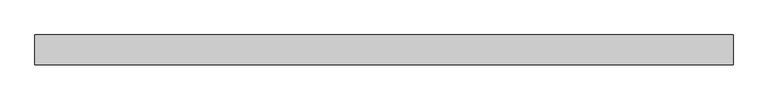
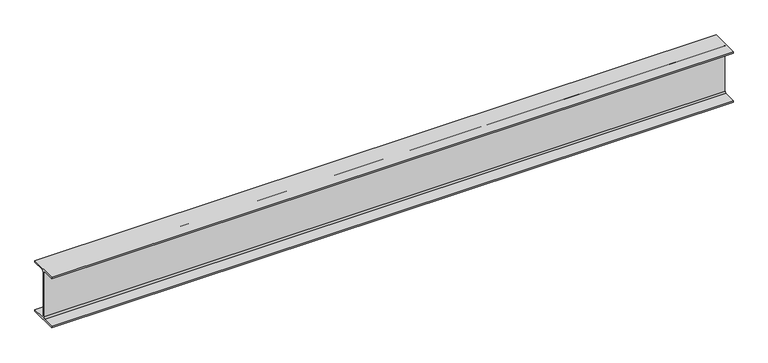
"""IFC4 building model written with IfcOpenShell, lengths in millimetres: beam geometry, Steel Beam_H-KSD3502 : H_SB_ASB_H-250x125x6x9."""

import ifcopenshell
import ifcopenshell.guid

model = None  # the IFC model being written
_history = None  # IfcOwnerHistory: only IFC2X3 demands one
_inside = {}  # id of a spatial element -> (the spatial element, [elements in it])
_under = {}  # id of a project, library or spatial element -> (it, [spatial elements below it])
_declared = {}  # id of a project -> (the project, [libraries it declares])
_typed = {}  # id of a type object -> (the type object, [elements of that type])
_made_of = {}  # id of a material, layer set ... -> (it, [elements and type objects made of it])


def new_model(schema):
    """Start an empty IFC model of exactly this schema.

    Asked for "IFC4X3", IfcOpenShell would pick the latest addendum, in which some entities
    have other attributes; the version numbers below select the first issue.
    IFC2X3 requires an IfcOwnerHistory on every rooted entity: one is made here for all.
    """
    global model, _history
    if schema == "IFC4X3":
        model = ifcopenshell.file(schema_version=(4, 3, 0, 0))
    else:
        model = ifcopenshell.file(schema=schema)
    _inside.clear()
    _under.clear()
    _declared.clear()
    _typed.clear()
    _made_of.clear()
    _history = None
    if model.schema == "IFC2X3":
        org = make("IfcOrganization", Name="unknown")
        user = make(
            "IfcPersonAndOrganization",
            ThePerson=make("IfcPerson", FamilyName="unknown"),
            TheOrganization=org,
        )
        app = make(
            "IfcApplication",
            ApplicationDeveloper=org,
            Version="unknown",
            ApplicationFullName="unknown",
            ApplicationIdentifier="unknown",
        )
        _history = make(
            "IfcOwnerHistory",
            OwningUser=user,
            OwningApplication=app,
            ChangeAction="ADDED",
            CreationDate=0,
        )
    return model


def make(cls, **values):
    """One entity of the class cls with the attributes given. An attribute that is None is left unset."""
    return model.create_entity(
        cls, **{name: value for name, value in values.items() if value is not None}
    )


def rooted(cls, **values):
    """An entity with a GlobalId (a new one), such as an element, a storey or a relation."""
    return make(cls, GlobalId=ifcopenshell.guid.new(), OwnerHistory=_history, **values)


def si_unit(unit_type, name, prefix=None):
    """IfcSIUnit, for example si_unit("LENGTHUNIT", "METRE", prefix="MILLI")."""
    return make("IfcSIUnit", UnitType=unit_type, Prefix=prefix, Name=name)


def assignment(units):
    """IfcUnitAssignment: the units of a project."""
    return None if units is None else make("IfcUnitAssignment", Units=units)


def point(xyz):
    """IfcCartesianPoint."""
    return None if xyz is None else make("IfcCartesianPoint", Coordinates=xyz)


def direction(xyz):
    """IfcDirection."""
    return None if xyz is None else make("IfcDirection", DirectionRatios=xyz)


def frame(location, z_axis=None, x_axis=None):
    """IfcAxis2Placement3D, a coordinate frame: its origin and axes. An axis left out is left unset."""
    return make(
        "IfcAxis2Placement3D",
        Location=point(location),
        Axis=direction(z_axis),
        RefDirection=direction(x_axis),
    )


def frame_2d(location, x_axis=None):
    """IfcAxis2Placement2D, a coordinate frame in the plane: its origin and x axis."""
    return make(
        "IfcAxis2Placement2D", Location=point(location), RefDirection=direction(x_axis)
    )


def origin():
    """The frame at (0, 0, 0) with its axes left unset."""
    return frame((0.0, 0.0, 0.0))


def place(relative_to, where):
    """IfcLocalPlacement: puts the frame where relative to a parent placement (None: the world)."""
    return make(
        "IfcLocalPlacement", PlacementRelTo=relative_to, RelativePlacement=where
    )


def context(
    kind, dimensions, precision=None, world=None, true_north=None, identifier=None
):
    """IfcGeometricRepresentationContext, for example the 3D "Model" context."""
    return make(
        "IfcGeometricRepresentationContext",
        ContextIdentifier=identifier,
        ContextType=kind,
        CoordinateSpaceDimension=dimensions,
        Precision=precision,
        WorldCoordinateSystem=world,
        TrueNorth=true_north,
    )


def project(units=None, contexts=None):
    """IfcProject with its units and contexts."""
    return rooted(
        "IfcProject",
        Name="project",
        RepresentationContexts=contexts,
        UnitsInContext=assignment(units),
    )


def spatial(cls, under=None, at=None, **own):
    """A site, building, storey or space (cls), placed at a placement, below another one or the project."""
    s = rooted(cls, ObjectPlacement=at, **own)
    if under is not None:
        _under.setdefault(under.id(), (under, []))[1].append(s)
    return s


def polyline(points):
    """IfcPolyline through the points."""
    return make("IfcPolyline", Points=[point(p) for p in points])


def circle_curve(where, radius):
    """IfcCircle in the frame where."""
    return make("IfcCircle", Position=where, Radius=radius)


def trimmed(basis, trim1, trim2, sense, master):
    """IfcTrimmedCurve: the piece of a basis curve between two trims."""
    return make(
        "IfcTrimmedCurve",
        BasisCurve=basis,
        Trim1=trim1,
        Trim2=trim2,
        SenseAgreement=sense,
        MasterRepresentation=master,
    )


def segment(curve, same_sense, transition):
    """IfcCompositeCurveSegment."""
    return make(
        "IfcCompositeCurveSegment",
        Transition=transition,
        SameSense=same_sense,
        ParentCurve=curve,
    )


def composite_curve(segments, self_intersect=None):
    """IfcCompositeCurve: segments joined end to end."""
    return make("IfcCompositeCurve", Segments=segments, SelfIntersect=self_intersect)


def outline(outer, holes=None, kind="AREA"):
    """IfcArbitraryClosedProfileDef: a profile drawn as a closed curve; with holes, ...WithVoids."""
    if holes is None:
        return make("IfcArbitraryClosedProfileDef", ProfileType=kind, OuterCurve=outer)
    return make(
        "IfcArbitraryProfileDefWithVoids",
        ProfileType=kind,
        OuterCurve=outer,
        InnerCurves=holes,
    )


def extrude(swept, where, along, depth):
    """IfcExtrudedAreaSolid: the profile swept, set in the frame where, extruded along a direction by depth."""
    return make(
        "IfcExtrudedAreaSolid",
        SweptArea=swept,
        Position=where,
        ExtrudedDirection=direction(along),
        Depth=depth,
    )


def shape(context_of_items, identifier, shape_type, items):
    """IfcShapeRepresentation: the items that make up one representation, for example the "Body"."""
    return make(
        "IfcShapeRepresentation",
        ContextOfItems=context_of_items,
        RepresentationIdentifier=identifier,
        RepresentationType=shape_type,
        Items=items,
    )


def source(mapping_origin, context_of_items, identifier, shape_type, items):
    """IfcRepresentationMap: a shape defined once, which mapped items show again and again."""
    return make(
        "IfcRepresentationMap",
        MappingOrigin=mapping_origin,
        MappedRepresentation=shape(context_of_items, identifier, shape_type, items),
    )


def transform(
    local_origin,
    x_axis=None,
    y_axis=None,
    z_axis=None,
    scale=None,
    scale2=None,
    scale3=None,
    uniform=True,
):
    """IfcCartesianTransformationOperator3D, or its non-uniform kind. x_axis, y_axis, z_axis: its Axis1, 2, 3."""
    if uniform:
        return make(
            "IfcCartesianTransformationOperator3D",
            Axis1=direction(x_axis),
            Axis2=direction(y_axis),
            LocalOrigin=point(local_origin),
            Scale=scale,
            Axis3=direction(z_axis),
        )
    return make(
        "IfcCartesianTransformationOperator3DnonUniform",
        Axis1=direction(x_axis),
        Axis2=direction(y_axis),
        LocalOrigin=point(local_origin),
        Scale=scale,
        Axis3=direction(z_axis),
        Scale2=scale2,
        Scale3=scale3,
    )


def mapped(mapping_source, mapping_target):
    """IfcMappedItem: shows the shape of a source again, moved by a transform."""
    return make(
        "IfcMappedItem", MappingSource=mapping_source, MappingTarget=mapping_target
    )


def made_of(thing, what):
    """Note that an element or type object is made of a material, layer set ...; save() writes the relation."""
    if what is not None:
        _made_of.setdefault(what.id(), (what, []))[1].append(thing)
    return thing


def element(
    cls,
    number,
    at=None,
    inside=None,
    cuts=None,
    type_object=None,
    material=None,
    context=None,
    identifier="Body",
    shape_type=None,
    held_by="IfcProductDefinitionShape",
    body=None,
    shapes=None,
    **own,
):
    """One element of the class cls, such as IfcWall. Its Tag is "e" and its number.

    at: its placement. inside: the storey or other place that contains it. cuts: it is an
    opening in that element (IfcRelVoidsElement). A single representation is given by context,
    identifier, shape_type and body (its items); several are given by shapes. held_by: the class
    of the entity that holds the representations. save() writes the other relations.
    """
    e = rooted(cls, Tag="e%d" % number, ObjectPlacement=at, **own)
    if body is not None:
        shapes = [shape(context, identifier, shape_type, body)]
    if shapes is not None:
        e.Representation = make(held_by, Representations=shapes)
    if inside is not None:
        _inside.setdefault(inside.id(), (inside, []))[1].append(e)
    if cuts is not None:
        rooted(
            "IfcRelVoidsElement", RelatingBuildingElement=cuts, RelatedOpeningElement=e
        )
    if type_object is not None:
        _typed.setdefault(type_object.id(), (type_object, []))[1].append(e)
    return made_of(e, material)


def aggregate(whole, parts):
    """IfcRelAggregates: a whole, such as a stair, and the parts it consists of."""
    return rooted("IfcRelAggregates", RelatingObject=whole, RelatedObjects=parts)


def save(model, path):
    """Write the relations noted so far, then the file.

    IfcRelAggregates (storeys below a building ...), IfcRelContainedInSpatialStructure (elements
    in a storey), IfcRelDefinesByType, IfcRelAssociatesMaterial and IfcRelDeclares: one each for
    every whole, place, type object, material and project.
    """
    for whole, parts in _under.values():
        aggregate(whole, parts)
    for where, things in _inside.values():
        rooted(
            "IfcRelContainedInSpatialStructure",
            RelatedElements=things,
            RelatingStructure=where,
        )
    for kind, things in _typed.values():
        rooted("IfcRelDefinesByType", RelatedObjects=things, RelatingType=kind)
    for what, things in _made_of.values():
        rooted("IfcRelAssociatesMaterial", RelatedObjects=things, RelatingMaterial=what)
    for by, libraries in _declared.values():
        rooted("IfcRelDeclares", RelatingContext=by, RelatedDefinitions=libraries)
    model.write(path)


def beam_8105422e(model_context):
    return source(origin(), model_context, "Body", "SweptSolid", [
        extrude(outline(composite_curve([segment(polyline([(82.5, -141.5), (82.5, -151.7), (-82.5, -151.7), (-82.5, -141.5), (-11.9, -141.5)]), True, "CONTINUOUS"), segment(trimmed(circle_curve(frame_2d((-11.9, -132.6)), 8.9), [point((-11.9, -141.5))], [point((-3.0, -132.6))], True, "CARTESIAN"), True, "CONTINUOUS"), segment(polyline([(-3.0, -132.6), (-3.0, 132.6)]), True, "CONTINUOUS"), segment(trimmed(circle_curve(frame_2d((-11.9, 132.6)), 8.9), [point((-3.0, 132.6))], [point((-11.9, 141.5))], True, "CARTESIAN"), True, "CONTINUOUS"), segment(polyline([(-11.9, 141.5), (-82.5, 141.5), (-82.5, 151.7), (82.5, 151.7), (82.5, 141.5), (11.9, 141.5)]), True, "CONTINUOUS"), segment(trimmed(circle_curve(frame_2d((11.9, 132.6)), 8.9), [point((11.9, 141.5))], [point((3.0, 132.6))], True, "CARTESIAN"), True, "CONTINUOUS"), segment(polyline([(3.0, 132.6), (3.0, -132.6)]), True, "CONTINUOUS"), segment(trimmed(circle_curve(frame_2d((11.9, -132.6)), 8.9), [point((3.0, -132.6))], [point((11.9, -141.5))], True, "CARTESIAN"), True, "CONTINUOUS"), segment(polyline([(11.9, -141.5), (82.5, -141.5)]), True, "CONTINUOUS")], self_intersect=False)), frame((-2029.8, 0.0, 0.0), z_axis=(1.0, 0.0, 0.0), x_axis=(0.0, 1.0, 0.0)), (0.0, 0.0, 1.0), 3859.8829189),
    ])


if __name__ == "__main__":
    model = new_model("IFC4")
    model_context = context("Model", 3, world=origin())
    ifc_project = project(units=[si_unit("LENGTHUNIT", "METRE", prefix="MILLI")], contexts=[model_context])
    site = spatial("IfcSite", under=ifc_project)
    building = spatial("IfcBuilding", under=site)
    placement = place(None, origin())
    beam_shape = beam_8105422e(model_context)
    element("IfcBeam", 1, ObjectType="Steel Beam_H-KSD3502 : H_SB_ASB_H-250x125x6x9", at=placement, inside=building, context=model_context, shape_type="MappedRepresentation", body=[
        mapped(beam_shape, transform((0.0, 0.0, 0.0), x_axis=(1.0, 0.0, 0.0), y_axis=(0.0, 1.0, 0.0), z_axis=(0.0, 0.0, 1.0))),
    ])
    save(model, "model.ifc")

# Revit data of these elements
# Type "Steel Beam_H-KSD3502 : H_SB_ASB_H-250x125x6x9"
#   Width = 12.5 cm
#   Web Thickness = 0.6 cm
#   Web Fillet = 1.2 cm
#   Warping Constant = 42539.8 cm⁶
#   Torsional Moment of Inertia = 7.8102 cm⁴
#   Torsional Modulus = 1.0 cm³
#   Section Area = 37.66 cm²
#   Plastic Modulus weak axis = 73.1 cm³
#   Plastic Modulus strong axis = 366.0 cm³
#   Perimeter = 0.97 m²/m
#   Nominal Weight = 29.60 kgf/m
#   Moment of Inertia weak axis = 294.00 cm⁴
#   Moment of Inertia strong axis = 4050.00 cm⁴
#   Height = 25.0 cm
#   Flange Thickness = 0.9 cm
#   Elastic Modulus weak axis = 47.0 cm³
#   Elastic Modulus strong axis = 324.0 cm³
#   Centroid Vertical = 12.5 cm
#   Centroid Horizontal = 6.25 cm
#   Length [instance default] = 1.5240 m
#   Structural Material [instance default] = Steel, 45-345
#   Assembly Code = ""
# Element 1 (IfcBeam, "Steel Beam_H-KSD3502 : H_SB_ASB_H-250x125x6x9")
#   Structural Material = none
# Materials
#   "Steel, 45-345": class "Metal", colour RGB 189 187 185, transparency 0, Description = "Steel 345 MPa", Cost = 0
